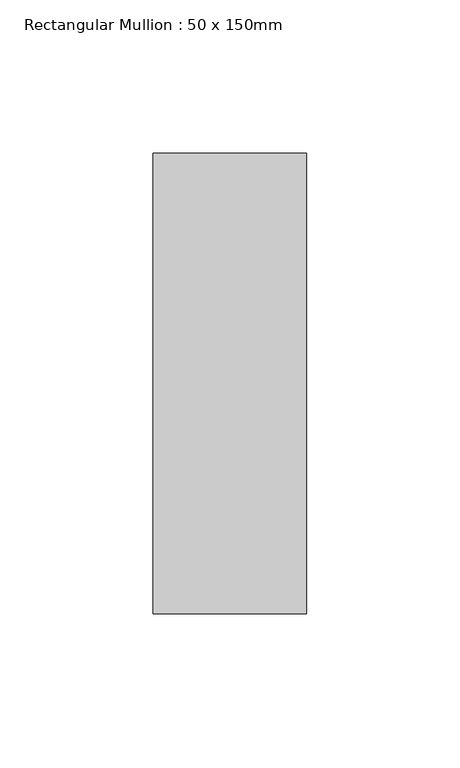
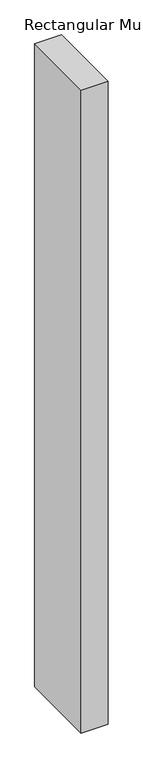
"""IFC4 building model written with IfcOpenShell, lengths in millimetres: member geometry, Rectangular Mullion : 50 x 150mm."""

from ifc_helpers import new_model, si_unit, frame, origin, place, context, project, spatial, polyline, outline, extrude, source, transform, mapped, element, save


def rectangular_mullion_50_x_150mm_58a8c50d(model_context):
    return source(origin(), model_context, "Body", "SweptSolid", [
        extrude(outline(polyline([(25.0, 75.0), (25.0, -75.0), (-25.0, -75.0), (-25.0, 75.0), (25.0, 75.0)])), frame((0.0, 0.0, -1266.108271), z_axis=(0.0, 0.0, 1.0), x_axis=(1.0, 0.0, 0.0)), (0.0, 0.0, 1.0), 1266.108271),
    ])


if __name__ == "__main__":
    model = new_model("IFC4")
    model_context = context("Model", 3, world=origin())
    ifc_project = project(units=[si_unit("LENGTHUNIT", "METRE", prefix="MILLI")], contexts=[model_context])
    site = spatial("IfcSite", under=ifc_project)
    building = spatial("IfcBuilding", under=site)
    placement = place(None, origin())
    rectangular_mullion_50_x_150mm_shape = rectangular_mullion_50_x_150mm_58a8c50d(model_context)
    element("IfcMember", 1, ObjectType="Rectangular Mullion : 50 x 150mm", at=placement, inside=building, context=model_context, shape_type="MappedRepresentation", body=[
        mapped(rectangular_mullion_50_x_150mm_shape, transform((0.0, 0.0, 0.0), x_axis=(1.0, 0.0, 0.0), y_axis=(0.0, 1.0, 0.0), z_axis=(0.0, 0.0, 1.0))),
    ])
    save(model, "model.ifc")

# Revit data of these elements
# Type "Rectangular Mullion : 50 x 150mm"
#   built-in parameter 1007304 = 0.492126 (stored number, unit not read)
#   built-in parameter 1007301 = 0.082021 (stored number, unit not read)
#   built-in parameter 1007300 = 0.082021 (stored number, unit not read)
# Element 1 (IfcMember, "Rectangular Mullion : 50 x 150mm")
#   Materials on its faces: "Aluminium"
# Materials
#   "Aluminium": class "Metal", colour RGB 247 247 247, transparency 0, Description = "Aluminium 6061", Cost = 0
